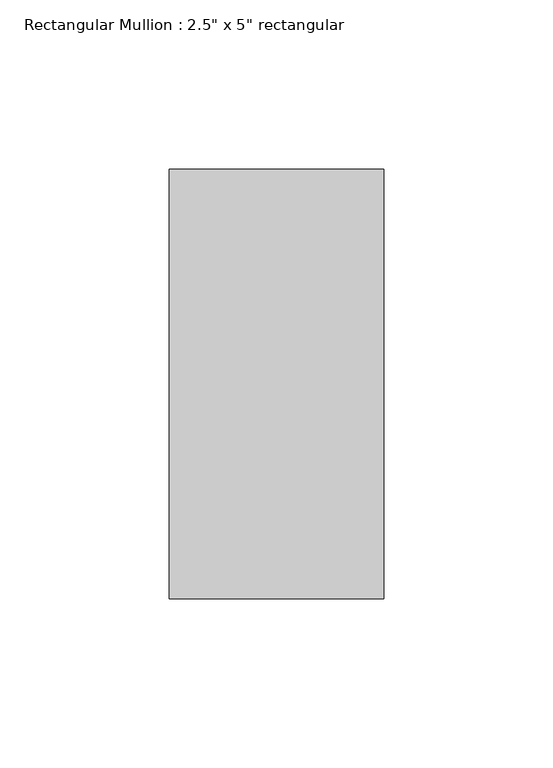
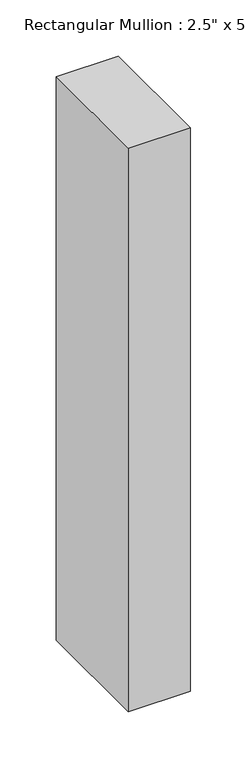
"""IFC4 building model written with IfcOpenShell, lengths in millimetres: member geometry."""

import ifcopenshell
import ifcopenshell.guid

model = None  # the IFC model being written
_history = None  # IfcOwnerHistory: only IFC2X3 demands one
_inside = {}  # id of a spatial element -> (the spatial element, [elements in it])
_under = {}  # id of a project, library or spatial element -> (it, [spatial elements below it])
_declared = {}  # id of a project -> (the project, [libraries it declares])
_typed = {}  # id of a type object -> (the type object, [elements of that type])
_made_of = {}  # id of a material, layer set ... -> (it, [elements and type objects made of it])


def new_model(schema):
    """Start an empty IFC model of exactly this schema.

    Asked for "IFC4X3", IfcOpenShell would pick the latest addendum, in which some entities
    have other attributes; the version numbers below select the first issue.
    IFC2X3 requires an IfcOwnerHistory on every rooted entity: one is made here for all.
    """
    global model, _history
    if schema == "IFC4X3":
        model = ifcopenshell.file(schema_version=(4, 3, 0, 0))
    else:
        model = ifcopenshell.file(schema=schema)
    _inside.clear()
    _under.clear()
    _declared.clear()
    _typed.clear()
    _made_of.clear()
    _history = None
    if model.schema == "IFC2X3":
        org = make("IfcOrganization", Name="unknown")
        user = make(
            "IfcPersonAndOrganization",
            ThePerson=make("IfcPerson", FamilyName="unknown"),
            TheOrganization=org,
        )
        app = make(
            "IfcApplication",
            ApplicationDeveloper=org,
            Version="unknown",
            ApplicationFullName="unknown",
            ApplicationIdentifier="unknown",
        )
        _history = make(
            "IfcOwnerHistory",
            OwningUser=user,
            OwningApplication=app,
            ChangeAction="ADDED",
            CreationDate=0,
        )
    return model


def make(cls, **values):
    """One entity of the class cls with the attributes given. An attribute that is None is left unset."""
    return model.create_entity(
        cls, **{name: value for name, value in values.items() if value is not None}
    )


def rooted(cls, **values):
    """An entity with a GlobalId (a new one), such as an element, a storey or a relation."""
    return make(cls, GlobalId=ifcopenshell.guid.new(), OwnerHistory=_history, **values)


def si_unit(unit_type, name, prefix=None):
    """IfcSIUnit, for example si_unit("LENGTHUNIT", "METRE", prefix="MILLI")."""
    return make("IfcSIUnit", UnitType=unit_type, Prefix=prefix, Name=name)


def assignment(units):
    """IfcUnitAssignment: the units of a project."""
    return None if units is None else make("IfcUnitAssignment", Units=units)


def point(xyz):
    """IfcCartesianPoint."""
    return None if xyz is None else make("IfcCartesianPoint", Coordinates=xyz)


def direction(xyz):
    """IfcDirection."""
    return None if xyz is None else make("IfcDirection", DirectionRatios=xyz)


def frame(location, z_axis=None, x_axis=None):
    """IfcAxis2Placement3D, a coordinate frame: its origin and axes. An axis left out is left unset."""
    return make(
        "IfcAxis2Placement3D",
        Location=point(location),
        Axis=direction(z_axis),
        RefDirection=direction(x_axis),
    )


def origin():
    """The frame at (0, 0, 0) with its axes left unset."""
    return frame((0.0, 0.0, 0.0))


def place(relative_to, where):
    """IfcLocalPlacement: puts the frame where relative to a parent placement (None: the world)."""
    return make(
        "IfcLocalPlacement", PlacementRelTo=relative_to, RelativePlacement=where
    )


def context(
    kind, dimensions, precision=None, world=None, true_north=None, identifier=None
):
    """IfcGeometricRepresentationContext, for example the 3D "Model" context."""
    return make(
        "IfcGeometricRepresentationContext",
        ContextIdentifier=identifier,
        ContextType=kind,
        CoordinateSpaceDimension=dimensions,
        Precision=precision,
        WorldCoordinateSystem=world,
        TrueNorth=true_north,
    )


def project(units=None, contexts=None):
    """IfcProject with its units and contexts."""
    return rooted(
        "IfcProject",
        Name="project",
        RepresentationContexts=contexts,
        UnitsInContext=assignment(units),
    )


def spatial(cls, under=None, at=None, **own):
    """A site, building, storey or space (cls), placed at a placement, below another one or the project."""
    s = rooted(cls, ObjectPlacement=at, **own)
    if under is not None:
        _under.setdefault(under.id(), (under, []))[1].append(s)
    return s


def polyline(points):
    """IfcPolyline through the points."""
    return make("IfcPolyline", Points=[point(p) for p in points])


def outline(outer, holes=None, kind="AREA"):
    """IfcArbitraryClosedProfileDef: a profile drawn as a closed curve; with holes, ...WithVoids."""
    if holes is None:
        return make("IfcArbitraryClosedProfileDef", ProfileType=kind, OuterCurve=outer)
    return make(
        "IfcArbitraryProfileDefWithVoids",
        ProfileType=kind,
        OuterCurve=outer,
        InnerCurves=holes,
    )


def extrude(swept, where, along, depth):
    """IfcExtrudedAreaSolid: the profile swept, set in the frame where, extruded along a direction by depth."""
    return make(
        "IfcExtrudedAreaSolid",
        SweptArea=swept,
        Position=where,
        ExtrudedDirection=direction(along),
        Depth=depth,
    )


def shape(context_of_items, identifier, shape_type, items):
    """IfcShapeRepresentation: the items that make up one representation, for example the "Body"."""
    return make(
        "IfcShapeRepresentation",
        ContextOfItems=context_of_items,
        RepresentationIdentifier=identifier,
        RepresentationType=shape_type,
        Items=items,
    )


def source(mapping_origin, context_of_items, identifier, shape_type, items):
    """IfcRepresentationMap: a shape defined once, which mapped items show again and again."""
    return make(
        "IfcRepresentationMap",
        MappingOrigin=mapping_origin,
        MappedRepresentation=shape(context_of_items, identifier, shape_type, items),
    )


def transform(
    local_origin,
    x_axis=None,
    y_axis=None,
    z_axis=None,
    scale=None,
    scale2=None,
    scale3=None,
    uniform=True,
):
    """IfcCartesianTransformationOperator3D, or its non-uniform kind. x_axis, y_axis, z_axis: its Axis1, 2, 3."""
    if uniform:
        return make(
            "IfcCartesianTransformationOperator3D",
            Axis1=direction(x_axis),
            Axis2=direction(y_axis),
            LocalOrigin=point(local_origin),
            Scale=scale,
            Axis3=direction(z_axis),
        )
    return make(
        "IfcCartesianTransformationOperator3DnonUniform",
        Axis1=direction(x_axis),
        Axis2=direction(y_axis),
        LocalOrigin=point(local_origin),
        Scale=scale,
        Axis3=direction(z_axis),
        Scale2=scale2,
        Scale3=scale3,
    )


def mapped(mapping_source, mapping_target):
    """IfcMappedItem: shows the shape of a source again, moved by a transform."""
    return make(
        "IfcMappedItem", MappingSource=mapping_source, MappingTarget=mapping_target
    )


def made_of(thing, what):
    """Note that an element or type object is made of a material, layer set ...; save() writes the relation."""
    if what is not None:
        _made_of.setdefault(what.id(), (what, []))[1].append(thing)
    return thing


def element(
    cls,
    number,
    at=None,
    inside=None,
    cuts=None,
    type_object=None,
    material=None,
    context=None,
    identifier="Body",
    shape_type=None,
    held_by="IfcProductDefinitionShape",
    body=None,
    shapes=None,
    **own,
):
    """One element of the class cls, such as IfcWall. Its Tag is "e" and its number.

    at: its placement. inside: the storey or other place that contains it. cuts: it is an
    opening in that element (IfcRelVoidsElement). A single representation is given by context,
    identifier, shape_type and body (its items); several are given by shapes. held_by: the class
    of the entity that holds the representations. save() writes the other relations.
    """
    e = rooted(cls, Tag="e%d" % number, ObjectPlacement=at, **own)
    if body is not None:
        shapes = [shape(context, identifier, shape_type, body)]
    if shapes is not None:
        e.Representation = make(held_by, Representations=shapes)
    if inside is not None:
        _inside.setdefault(inside.id(), (inside, []))[1].append(e)
    if cuts is not None:
        rooted(
            "IfcRelVoidsElement", RelatingBuildingElement=cuts, RelatedOpeningElement=e
        )
    if type_object is not None:
        _typed.setdefault(type_object.id(), (type_object, []))[1].append(e)
    return made_of(e, material)


def aggregate(whole, parts):
    """IfcRelAggregates: a whole, such as a stair, and the parts it consists of."""
    return rooted("IfcRelAggregates", RelatingObject=whole, RelatedObjects=parts)


def save(model, path):
    """Write the relations noted so far, then the file.

    IfcRelAggregates (storeys below a building ...), IfcRelContainedInSpatialStructure (elements
    in a storey), IfcRelDefinesByType, IfcRelAssociatesMaterial and IfcRelDeclares: one each for
    every whole, place, type object, material and project.
    """
    for whole, parts in _under.values():
        aggregate(whole, parts)
    for where, things in _inside.values():
        rooted(
            "IfcRelContainedInSpatialStructure",
            RelatedElements=things,
            RelatingStructure=where,
        )
    for kind, things in _typed.values():
        rooted("IfcRelDefinesByType", RelatedObjects=things, RelatingType=kind)
    for what, things in _made_of.values():
        rooted("IfcRelAssociatesMaterial", RelatedObjects=things, RelatingMaterial=what)
    for by, libraries in _declared.values():
        rooted("IfcRelDeclares", RelatingContext=by, RelatedDefinitions=libraries)
    model.write(path)


def member_47bfaf8a(model_context):
    return source(origin(), model_context, "Body", "SweptSolid", [
        extrude(outline(polyline([(0.0, 63.5), (0.0, -63.5), (-63.5, -63.5), (-63.5, 63.5), (0.0, 63.5)])), frame((0.0, 0.0, -609.6), z_axis=(0.0, 0.0, 1.0), x_axis=(1.0, 0.0, 0.0)), (0.0, 0.0, 1.0), 609.6),
    ])


if __name__ == "__main__":
    model = new_model("IFC4")
    model_context = context("Model", 3, world=origin())
    ifc_project = project(units=[si_unit("LENGTHUNIT", "METRE", prefix="MILLI")], contexts=[model_context])
    site = spatial("IfcSite", under=ifc_project)
    building = spatial("IfcBuilding", under=site)
    placement = place(None, origin())
    member_shape = member_47bfaf8a(model_context)
    element("IfcMember", 1, ObjectType="Rectangular Mullion : 2.5\" x 5\" rectangular", at=placement, inside=building, context=model_context, shape_type="MappedRepresentation", body=[
        mapped(member_shape, transform((0.0, 0.0, 0.0), x_axis=(1.0, 0.0, 0.0), y_axis=(0.0, 1.0, 0.0), z_axis=(0.0, 0.0, 1.0))),
    ])
    save(model, "model.ifc")

# Revit data of these elements
# Type "Rectangular Mullion : 2.5\" x 5\" rectangular"
#   built-in parameter 1007304 = 0.416667 (stored number, unit not read)
#   built-in parameter 1007301 = 0.104167 (stored number, unit not read)
#   built-in parameter 1007300 = 0.104167 (stored number, unit not read)
# Element 1 (IfcMember, "Rectangular Mullion : 2.5\" x 5\" rectangular")
#   Materials on its faces: "Aluminum"
# Materials
#   "Aluminum": class "Metal", colour RGB 247 247 247, transparency 0, Description = "Aluminum 6061", Cost = 0
